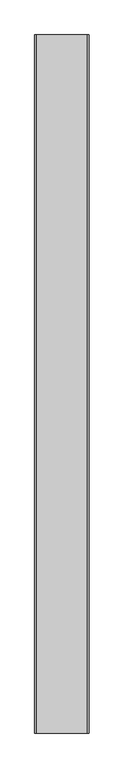
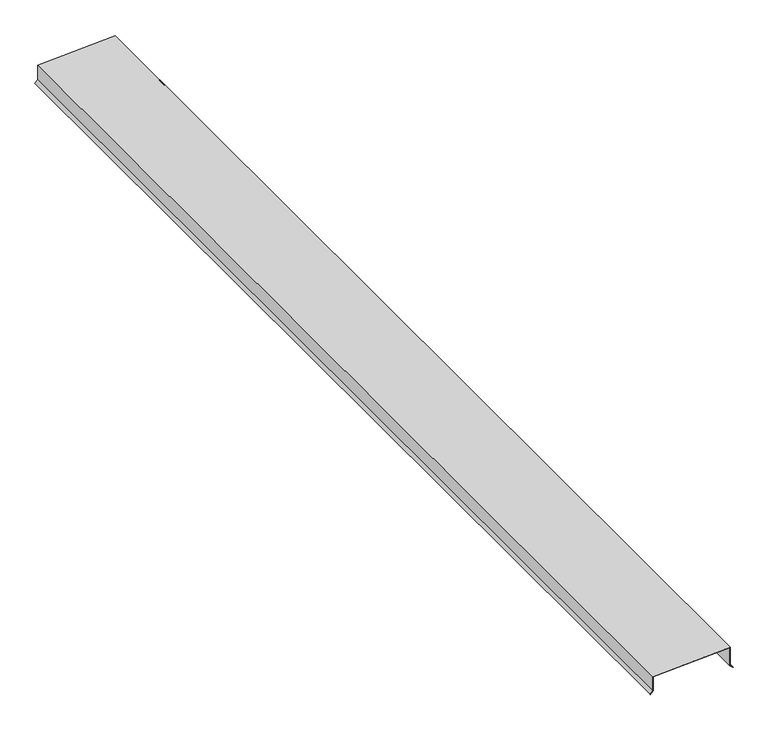
"""IFC4 building model written with IfcOpenShell, lengths in millimetres: proxy geometry, Generic Models 7:Generic Models 1:5:Generic Models 1:5 : Generic Models 7:Generic Models 1:337419:20 : Generic Models 7:Generic Models 1:5:Generic Models 1:5 : Generic Models 7:Generic Models 1:337419:311462."""

from ifc_helpers import new_model, si_unit, frame, origin, place, context, project, spatial, polyline, outline, extrude, source, transform, mapped, element, save


def generic_models_75ba2336(model_context):
    return source(origin(), model_context, "Body", "SweptSolid", [
        extrude(outline(polyline([(6099.8348677, 579418.8367239), (6188.1524863, 579418.8367239), (6169.5994773, 579064.8242239), (6099.8348677, 579064.8242239), (6087.1348677, 579052.1242239), (6086.0123357, 579053.246756), (6099.1773037, 579066.4117239), (6168.0929961, 579066.4117239), (6186.4796103, 579417.2492239), (6099.1773037, 579417.2492239), (6086.0123357, 579430.4141919), (6087.1348677, 579431.5367239), (6099.8348677, 579418.8367239)])), frame((0.0, -578718.1163842, 0.0), z_axis=(0.0, 1.0, 0.0), x_axis=(0.0, 0.0, 1.0)), (0.0, 0.0, 1.0), 4876.8),
    ])


if __name__ == "__main__":
    model = new_model("IFC4")
    model_context = context("Model", 3, world=origin())
    ifc_project = project(units=[si_unit("LENGTHUNIT", "METRE", prefix="MILLI")], contexts=[model_context])
    site = spatial("IfcSite", under=ifc_project)
    building = spatial("IfcBuilding", under=site)
    placement = place(None, origin())
    generic_models_shape = generic_models_75ba2336(model_context)
    element("IfcBuildingElementProxy", 1, Name="Generic Models 7:Generic Models 1:5:Generic Models 1:5 : Generic Models 7:Generic Models 1:337419:20 : Generic Models 7:Generic Models 1:5:Generic Models 1:5 : Generic Models 7:Generic Models 1:337419:311462", ObjectType="Generic Models 7:Generic Models 1:5:Generic Models 1:5 : Generic Models 7:Generic Models 1:337419:20 : Generic Models 7:Generic Models 1:5:Generic Models 1:5 : Generic Models 7:Generic Models 1:337419:311462", at=placement, inside=building, context=model_context, shape_type="MappedRepresentation", body=[
        mapped(generic_models_shape, transform((0.0, 0.0, 0.0), x_axis=(1.0, 0.0, 0.0), y_axis=(0.0, 1.0, 0.0), z_axis=(0.0, 0.0, 1.0))),
    ])
    save(model, "model.ifc")

# Revit data of these elements
# Type "Generic Models 7:Generic Models 1:5:Generic Models 1:5 : Generic Models 7:Generic Models 1:337419:20 : Generic Models 7:Generic Models 1:5:Generic Models 1:5 : Generic Models 7:Generic Models 1:337419:311462"
#   NameOverride = "Generic Models 7:Generic Models 1:5:Generic Models 1:5 : Generic Models 7:Generic Models 1:337419:311462"
#   ObjectTypeOverride = "Generic Models 1:5 : Generic Models 7:Generic Models 1:337419"
#   Reference = "Generic Models 1"
#   Tag = "311462"
# Element 1 (IfcBuildingElementProxy, "Generic Models 7:Generic Models 1:5:Generic Models 1:5 : Generic Models 7:Generic Models 1:337419:20 : Generic Models 7:Generic Models 1:5:Generic Models 1:5 : Generic Models 7:Generic Models 1:337419:311462")
#   Materials on its faces: "SLOPED SHEET METAL COPING - (COLOR TO MATCH RESIN PANEL)"
# Materials
#   "SLOPED SHEET METAL COPING - (COLOR TO MATCH RESIN PANEL)": class "Generic", colour RGB 240 240 240, transparency 0, Keynote = "M07711300.01", Cost = 0
